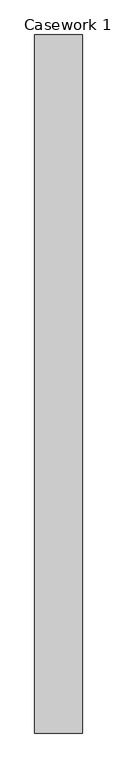
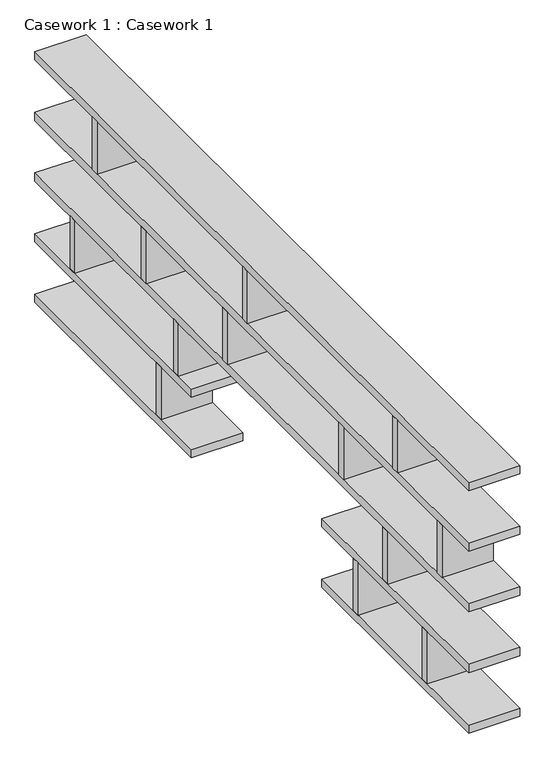
"""IFC4 building model written with IfcOpenShell, lengths in millimetres: furniture geometry, Casework 1 : Casework 1."""

from ifc_helpers import new_model, si_unit, frame, origin, place, context, project, spatial, polyline, outline, extrude, source, transform, mapped, element, save


def casework_1_casework_1_088f9a77(model_context):
    return source(origin(), model_context, "Body", "SweptSolid", [
        extrude(outline(polyline([(-8890.9168771, 3567.8656876), (-9195.7168771, 3567.8656876), (-9195.7168771, 3618.6656876), (-8890.9168771, 3618.6656876), (-8890.9168771, 3567.8656876)])), frame((0.0, 0.0, 4876.8), z_axis=(0.0, 0.0, 1.0), x_axis=(1.0, 0.0, 0.0)), (0.0, 0.0, 1.0), 330.2),
        extrude(outline(polyline([(-8890.9168771, 1535.8656876), (-9195.7168771, 1535.8656876), (-9195.7168771, 1586.6656876), (-8890.9168771, 1586.6656876), (-8890.9168771, 1535.8656876)])), frame((0.0, 0.0, 4876.8), z_axis=(0.0, 0.0, 1.0), x_axis=(1.0, 0.0, 0.0)), (0.0, 0.0, 1.0), 330.2),
        extrude(outline(polyline([(-8890.9168771, 824.6656876), (-9195.7168771, 824.6656876), (-9195.7168771, 875.4656876), (-8890.9168771, 875.4656876), (-8890.9168771, 824.6656876)])), frame((0.0, 0.0, 4876.8), z_axis=(0.0, 0.0, 1.0), x_axis=(1.0, 0.0, 0.0)), (0.0, 0.0, 1.0), 330.2),
        extrude(outline(polyline([(-8890.9168771, 4456.8656876), (-9195.7168771, 4456.8656876), (-9195.7168771, 4507.6656876), (-8890.9168771, 4507.6656876), (-8890.9168771, 4456.8656876)])), frame((0.0, 0.0, 5257.8), z_axis=(0.0, 0.0, 1.0), x_axis=(1.0, 0.0, 0.0)), (0.0, 0.0, 1.0), 330.2),
        extrude(outline(polyline([(-8890.9168771, 3390.0656876), (-9195.7168771, 3390.0656876), (-9195.7168771, 3440.8656876), (-8890.9168771, 3440.8656876), (-8890.9168771, 3390.0656876)])), frame((0.0, 0.0, 5257.8), z_axis=(0.0, 0.0, 1.0), x_axis=(1.0, 0.0, 0.0)), (0.0, 0.0, 1.0), 330.2),
        extrude(outline(polyline([(-8890.9168771, 1231.0656876), (-9195.7168771, 1231.0656876), (-9195.7168771, 1281.8656876), (-8890.9168771, 1281.8656876), (-8890.9168771, 1231.0656876)])), frame((0.0, 0.0, 5257.8), z_axis=(0.0, 0.0, 1.0), x_axis=(1.0, 0.0, 0.0)), (0.0, 0.0, 1.0), 330.2),
        extrude(outline(polyline([(-8890.9168771, 3720.2656876), (-9195.7168771, 3720.2656876), (-9195.7168771, 3771.0656876), (-8890.9168771, 3771.0656876), (-8890.9168771, 3720.2656876)])), frame((0.0, 0.0, 5638.8), z_axis=(0.0, 0.0, 1.0), x_axis=(1.0, 0.0, 0.0)), (0.0, 0.0, 1.0), 330.2),
        extrude(outline(polyline([(-8890.9168771, 2882.0656876), (-9195.7168771, 2882.0656876), (-9195.7168771, 2932.8656876), (-8890.9168771, 2932.8656876), (-8890.9168771, 2882.0656876)])), frame((0.0, 0.0, 5638.8), z_axis=(0.0, 0.0, 1.0), x_axis=(1.0, 0.0, 0.0)), (0.0, 0.0, 1.0), 330.2),
        extrude(outline(polyline([(-8890.9168771, 1688.2656876), (-9195.7168771, 1688.2656876), (-9195.7168771, 1739.0656876), (-8890.9168771, 1739.0656876), (-8890.9168771, 1688.2656876)])), frame((0.0, 0.0, 5638.8), z_axis=(0.0, 0.0, 1.0), x_axis=(1.0, 0.0, 0.0)), (0.0, 0.0, 1.0), 330.2),
        extrude(outline(polyline([(-8890.9168771, 672.2656876), (-9195.7168771, 672.2656876), (-9195.7168771, 723.0656876), (-8890.9168771, 723.0656876), (-8890.9168771, 672.2656876)])), frame((0.0, 0.0, 5638.8), z_axis=(0.0, 0.0, 1.0), x_axis=(1.0, 0.0, 0.0)), (0.0, 0.0, 1.0), 330.2),
        extrude(outline(polyline([(-8890.9168771, 4228.2656876), (-9195.7168771, 4228.2656876), (-9195.7168771, 4279.0656876), (-8890.9168771, 4279.0656876), (-8890.9168771, 4228.2656876)])), frame((0.0, 0.0, 6019.8), z_axis=(0.0, 0.0, 1.0), x_axis=(1.0, 0.0, 0.0)), (0.0, 0.0, 1.0), 330.2),
        extrude(outline(polyline([(-8890.9168771, 2678.8656876), (-9195.7168771, 2678.8656876), (-9195.7168771, 2729.6656876), (-8890.9168771, 2729.6656876), (-8890.9168771, 2678.8656876)])), frame((0.0, 0.0, 6019.8), z_axis=(0.0, 0.0, 1.0), x_axis=(1.0, 0.0, 0.0)), (0.0, 0.0, 1.0), 330.2),
        extrude(outline(polyline([(-8890.9168771, 1129.4656876), (-9195.7168771, 1129.4656876), (-9195.7168771, 1180.2656876), (-8890.9168771, 1180.2656876), (-8890.9168771, 1129.4656876)])), frame((0.0, 0.0, 6019.8), z_axis=(0.0, 0.0, 1.0), x_axis=(1.0, 0.0, 0.0)), (0.0, 0.0, 1.0), 330.2),
        extrude(outline(polyline([(-8890.9168771, 4869.4728535), (-8890.9168771, 399.0728535), (-9195.7168771, 399.0728535), (-9195.7168771, 4869.4728535), (-8890.9168771, 4869.4728535)])), frame((0.0, 0.0, 6350.0), z_axis=(0.0, 0.0, 1.0), x_axis=(1.0, 0.0, 0.0)), (0.0, 0.0, 1.0), 50.8),
        extrude(outline(polyline([(-8890.9168771, 399.0728535), (-9195.7168771, 399.0728535), (-9195.7168771, 1910.6585217), (-8890.9168771, 1910.6585217), (-8890.9168771, 399.0728535)])), frame((0.0, 0.0, 5207.0), z_axis=(0.0, 0.0, 1.0), x_axis=(1.0, 0.0, 0.0)), (0.0, 0.0, 1.0), 50.8),
        extrude(outline(polyline([(-8890.9168771, 399.0728535), (-9195.7168771, 399.0728535), (-9195.7168771, 1910.6585217), (-8890.9168771, 1910.6585217), (-8890.9168771, 399.0728535)])), frame((0.0, 0.0, 4826.0), z_axis=(0.0, 0.0, 1.0), x_axis=(1.0, 0.0, 0.0)), (0.0, 0.0, 1.0), 50.8),
        extrude(outline(polyline([(-8890.9168771, 4869.4728535), (-8890.9168771, 399.0728535), (-9195.7168771, 399.0728535), (-9195.7168771, 4869.4728535), (-8890.9168771, 4869.4728535)])), frame((0.0, 0.0, 5969.0), z_axis=(0.0, 0.0, 1.0), x_axis=(1.0, 0.0, 0.0)), (0.0, 0.0, 1.0), 50.8),
        extrude(outline(polyline([(-8890.9168771, 4869.4728535), (-8890.9168771, 399.0728535), (-9195.7168771, 399.0728535), (-9195.7168771, 4869.4728535), (-8890.9168771, 4869.4728535)])), frame((0.0, 0.0, 5588.0), z_axis=(0.0, 0.0, 1.0), x_axis=(1.0, 0.0, 0.0)), (0.0, 0.0, 1.0), 50.8),
        extrude(outline(polyline([(-8890.9168771, 4869.4728535), (-8890.9168771, 3256.2871852), (-9195.7168771, 3256.2871852), (-9195.7168771, 4869.4728535), (-8890.9168771, 4869.4728535)])), frame((0.0, 0.0, 5207.0), z_axis=(0.0, 0.0, 1.0), x_axis=(1.0, 0.0, 0.0)), (0.0, 0.0, 1.0), 50.8),
        extrude(outline(polyline([(-8890.9168771, 4869.4728535), (-8890.9168771, 3256.2871852), (-9195.7168771, 3256.2871852), (-9195.7168771, 4869.4728535), (-8890.9168771, 4869.4728535)])), frame((0.0, 0.0, 4826.0), z_axis=(0.0, 0.0, 1.0), x_axis=(1.0, 0.0, 0.0)), (0.0, 0.0, 1.0), 50.8),
    ])


if __name__ == "__main__":
    model = new_model("IFC4")
    model_context = context("Model", 3, world=origin())
    ifc_project = project(units=[si_unit("LENGTHUNIT", "METRE", prefix="MILLI")], contexts=[model_context])
    site = spatial("IfcSite", under=ifc_project)
    building = spatial("IfcBuilding", under=site)
    placement = place(None, origin())
    casework_1_casework_1_shape = casework_1_casework_1_088f9a77(model_context)
    element("IfcFurniture", 1, ObjectType="Casework 1 : Casework 1", at=placement, inside=building, context=model_context, shape_type="MappedRepresentation", body=[
        mapped(casework_1_casework_1_shape, transform((0.0, 0.0, 0.0), x_axis=(1.0, 0.0, 0.0), y_axis=(0.0, 1.0, 0.0), z_axis=(0.0, 0.0, 1.0))),
    ])
    save(model, "model.ifc")

# Revit data of these elements
# Project information
#   Project Issue Date = "12.12.2014"
#   Project Status = "Project Status"
#   Client Name = "Stephan & Brady"
#   Project Address = "Enter address here"
#   Project Name = "Stephan Brady - New Balcony"
#   Project Number = "Project Number"
# Element 1 (IfcFurniture, "Casework 1 : Casework 1")
#   Materials on its faces: "Countertop & Shelf"
# Materials
#   "Countertop & Shelf": class "Paint", colour RGB 76 54 29, transparency 0, Cost = 0
